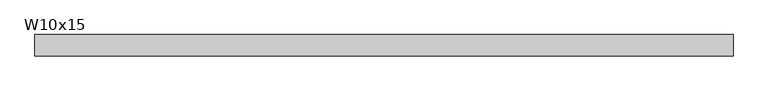
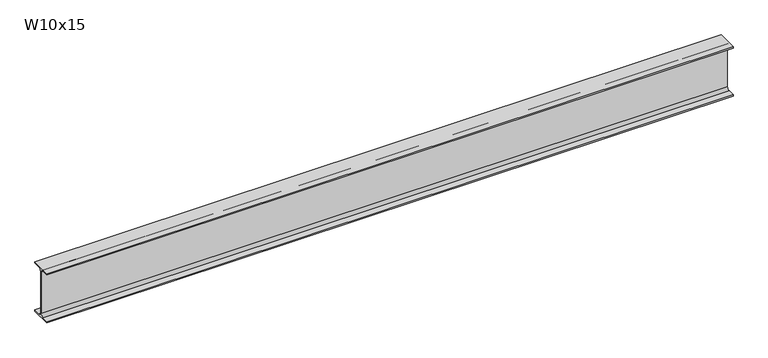
"""IFC4 building model written with IfcOpenShell, lengths in millimetres: beam geometry, RME W-Wide Flange : W10x15."""

import ifcopenshell
import ifcopenshell.guid

model = None  # the IFC model being written
_history = None  # IfcOwnerHistory: only IFC2X3 demands one
_inside = {}  # id of a spatial element -> (the spatial element, [elements in it])
_under = {}  # id of a project, library or spatial element -> (it, [spatial elements below it])
_declared = {}  # id of a project -> (the project, [libraries it declares])
_typed = {}  # id of a type object -> (the type object, [elements of that type])
_made_of = {}  # id of a material, layer set ... -> (it, [elements and type objects made of it])


def new_model(schema):
    """Start an empty IFC model of exactly this schema.

    Asked for "IFC4X3", IfcOpenShell would pick the latest addendum, in which some entities
    have other attributes; the version numbers below select the first issue.
    IFC2X3 requires an IfcOwnerHistory on every rooted entity: one is made here for all.
    """
    global model, _history
    if schema == "IFC4X3":
        model = ifcopenshell.file(schema_version=(4, 3, 0, 0))
    else:
        model = ifcopenshell.file(schema=schema)
    _inside.clear()
    _under.clear()
    _declared.clear()
    _typed.clear()
    _made_of.clear()
    _history = None
    if model.schema == "IFC2X3":
        org = make("IfcOrganization", Name="unknown")
        user = make(
            "IfcPersonAndOrganization",
            ThePerson=make("IfcPerson", FamilyName="unknown"),
            TheOrganization=org,
        )
        app = make(
            "IfcApplication",
            ApplicationDeveloper=org,
            Version="unknown",
            ApplicationFullName="unknown",
            ApplicationIdentifier="unknown",
        )
        _history = make(
            "IfcOwnerHistory",
            OwningUser=user,
            OwningApplication=app,
            ChangeAction="ADDED",
            CreationDate=0,
        )
    return model


def make(cls, **values):
    """One entity of the class cls with the attributes given. An attribute that is None is left unset."""
    return model.create_entity(
        cls, **{name: value for name, value in values.items() if value is not None}
    )


def rooted(cls, **values):
    """An entity with a GlobalId (a new one), such as an element, a storey or a relation."""
    return make(cls, GlobalId=ifcopenshell.guid.new(), OwnerHistory=_history, **values)


def si_unit(unit_type, name, prefix=None):
    """IfcSIUnit, for example si_unit("LENGTHUNIT", "METRE", prefix="MILLI")."""
    return make("IfcSIUnit", UnitType=unit_type, Prefix=prefix, Name=name)


def assignment(units):
    """IfcUnitAssignment: the units of a project."""
    return None if units is None else make("IfcUnitAssignment", Units=units)


def point(xyz):
    """IfcCartesianPoint."""
    return None if xyz is None else make("IfcCartesianPoint", Coordinates=xyz)


def direction(xyz):
    """IfcDirection."""
    return None if xyz is None else make("IfcDirection", DirectionRatios=xyz)


def frame(location, z_axis=None, x_axis=None):
    """IfcAxis2Placement3D, a coordinate frame: its origin and axes. An axis left out is left unset."""
    return make(
        "IfcAxis2Placement3D",
        Location=point(location),
        Axis=direction(z_axis),
        RefDirection=direction(x_axis),
    )


def frame_2d(location, x_axis=None):
    """IfcAxis2Placement2D, a coordinate frame in the plane: its origin and x axis."""
    return make(
        "IfcAxis2Placement2D", Location=point(location), RefDirection=direction(x_axis)
    )


def origin():
    """The frame at (0, 0, 0) with its axes left unset."""
    return frame((0.0, 0.0, 0.0))


def place(relative_to, where):
    """IfcLocalPlacement: puts the frame where relative to a parent placement (None: the world)."""
    return make(
        "IfcLocalPlacement", PlacementRelTo=relative_to, RelativePlacement=where
    )


def context(
    kind, dimensions, precision=None, world=None, true_north=None, identifier=None
):
    """IfcGeometricRepresentationContext, for example the 3D "Model" context."""
    return make(
        "IfcGeometricRepresentationContext",
        ContextIdentifier=identifier,
        ContextType=kind,
        CoordinateSpaceDimension=dimensions,
        Precision=precision,
        WorldCoordinateSystem=world,
        TrueNorth=true_north,
    )


def project(units=None, contexts=None):
    """IfcProject with its units and contexts."""
    return rooted(
        "IfcProject",
        Name="project",
        RepresentationContexts=contexts,
        UnitsInContext=assignment(units),
    )


def spatial(cls, under=None, at=None, **own):
    """A site, building, storey or space (cls), placed at a placement, below another one or the project."""
    s = rooted(cls, ObjectPlacement=at, **own)
    if under is not None:
        _under.setdefault(under.id(), (under, []))[1].append(s)
    return s


def polyline(points):
    """IfcPolyline through the points."""
    return make("IfcPolyline", Points=[point(p) for p in points])


def circle_curve(where, radius):
    """IfcCircle in the frame where."""
    return make("IfcCircle", Position=where, Radius=radius)


def trimmed(basis, trim1, trim2, sense, master):
    """IfcTrimmedCurve: the piece of a basis curve between two trims."""
    return make(
        "IfcTrimmedCurve",
        BasisCurve=basis,
        Trim1=trim1,
        Trim2=trim2,
        SenseAgreement=sense,
        MasterRepresentation=master,
    )


def segment(curve, same_sense, transition):
    """IfcCompositeCurveSegment."""
    return make(
        "IfcCompositeCurveSegment",
        Transition=transition,
        SameSense=same_sense,
        ParentCurve=curve,
    )


def composite_curve(segments, self_intersect=None):
    """IfcCompositeCurve: segments joined end to end."""
    return make("IfcCompositeCurve", Segments=segments, SelfIntersect=self_intersect)


def outline(outer, holes=None, kind="AREA"):
    """IfcArbitraryClosedProfileDef: a profile drawn as a closed curve; with holes, ...WithVoids."""
    if holes is None:
        return make("IfcArbitraryClosedProfileDef", ProfileType=kind, OuterCurve=outer)
    return make(
        "IfcArbitraryProfileDefWithVoids",
        ProfileType=kind,
        OuterCurve=outer,
        InnerCurves=holes,
    )


def extrude(swept, where, along, depth):
    """IfcExtrudedAreaSolid: the profile swept, set in the frame where, extruded along a direction by depth."""
    return make(
        "IfcExtrudedAreaSolid",
        SweptArea=swept,
        Position=where,
        ExtrudedDirection=direction(along),
        Depth=depth,
    )


def shape(context_of_items, identifier, shape_type, items):
    """IfcShapeRepresentation: the items that make up one representation, for example the "Body"."""
    return make(
        "IfcShapeRepresentation",
        ContextOfItems=context_of_items,
        RepresentationIdentifier=identifier,
        RepresentationType=shape_type,
        Items=items,
    )


def source(mapping_origin, context_of_items, identifier, shape_type, items):
    """IfcRepresentationMap: a shape defined once, which mapped items show again and again."""
    return make(
        "IfcRepresentationMap",
        MappingOrigin=mapping_origin,
        MappedRepresentation=shape(context_of_items, identifier, shape_type, items),
    )


def transform(
    local_origin,
    x_axis=None,
    y_axis=None,
    z_axis=None,
    scale=None,
    scale2=None,
    scale3=None,
    uniform=True,
):
    """IfcCartesianTransformationOperator3D, or its non-uniform kind. x_axis, y_axis, z_axis: its Axis1, 2, 3."""
    if uniform:
        return make(
            "IfcCartesianTransformationOperator3D",
            Axis1=direction(x_axis),
            Axis2=direction(y_axis),
            LocalOrigin=point(local_origin),
            Scale=scale,
            Axis3=direction(z_axis),
        )
    return make(
        "IfcCartesianTransformationOperator3DnonUniform",
        Axis1=direction(x_axis),
        Axis2=direction(y_axis),
        LocalOrigin=point(local_origin),
        Scale=scale,
        Axis3=direction(z_axis),
        Scale2=scale2,
        Scale3=scale3,
    )


def mapped(mapping_source, mapping_target):
    """IfcMappedItem: shows the shape of a source again, moved by a transform."""
    return make(
        "IfcMappedItem", MappingSource=mapping_source, MappingTarget=mapping_target
    )


def made_of(thing, what):
    """Note that an element or type object is made of a material, layer set ...; save() writes the relation."""
    if what is not None:
        _made_of.setdefault(what.id(), (what, []))[1].append(thing)
    return thing


def element(
    cls,
    number,
    at=None,
    inside=None,
    cuts=None,
    type_object=None,
    material=None,
    context=None,
    identifier="Body",
    shape_type=None,
    held_by="IfcProductDefinitionShape",
    body=None,
    shapes=None,
    **own,
):
    """One element of the class cls, such as IfcWall. Its Tag is "e" and its number.

    at: its placement. inside: the storey or other place that contains it. cuts: it is an
    opening in that element (IfcRelVoidsElement). A single representation is given by context,
    identifier, shape_type and body (its items); several are given by shapes. held_by: the class
    of the entity that holds the representations. save() writes the other relations.
    """
    e = rooted(cls, Tag="e%d" % number, ObjectPlacement=at, **own)
    if body is not None:
        shapes = [shape(context, identifier, shape_type, body)]
    if shapes is not None:
        e.Representation = make(held_by, Representations=shapes)
    if inside is not None:
        _inside.setdefault(inside.id(), (inside, []))[1].append(e)
    if cuts is not None:
        rooted(
            "IfcRelVoidsElement", RelatingBuildingElement=cuts, RelatedOpeningElement=e
        )
    if type_object is not None:
        _typed.setdefault(type_object.id(), (type_object, []))[1].append(e)
    return made_of(e, material)


def aggregate(whole, parts):
    """IfcRelAggregates: a whole, such as a stair, and the parts it consists of."""
    return rooted("IfcRelAggregates", RelatingObject=whole, RelatedObjects=parts)


def save(model, path):
    """Write the relations noted so far, then the file.

    IfcRelAggregates (storeys below a building ...), IfcRelContainedInSpatialStructure (elements
    in a storey), IfcRelDefinesByType, IfcRelAssociatesMaterial and IfcRelDeclares: one each for
    every whole, place, type object, material and project.
    """
    for whole, parts in _under.values():
        aggregate(whole, parts)
    for where, things in _inside.values():
        rooted(
            "IfcRelContainedInSpatialStructure",
            RelatedElements=things,
            RelatingStructure=where,
        )
    for kind, things in _typed.values():
        rooted("IfcRelDefinesByType", RelatedObjects=things, RelatingType=kind)
    for what, things in _made_of.values():
        rooted("IfcRelAssociatesMaterial", RelatedObjects=things, RelatingMaterial=what)
    for by, libraries in _declared.values():
        rooted("IfcRelDeclares", RelatingContext=by, RelatedDefinitions=libraries)
    model.write(path)


def w10x15_412ed89f(model_context):
    return source(origin(), model_context, "Body", "SweptSolid", [
        extrude(outline(composite_curve([segment(polyline([(50.8, -120.142), (50.8, -127.0), (-50.8, -127.0), (-50.8, -120.142), (-16.7005, -120.142)]), True, "CONTINUOUS"), segment(trimmed(circle_curve(frame_2d((-16.7005, -106.3625)), 13.7795), [point((-16.7005, -120.142))], [point((-2.921, -106.3625))], True, "CARTESIAN"), True, "CONTINUOUS"), segment(polyline([(-2.921, -106.3625), (-2.921, 106.3625)]), True, "CONTINUOUS"), segment(trimmed(circle_curve(frame_2d((-16.7005, 106.3625)), 13.7795), [point((-2.921, 106.3625))], [point((-16.7005, 120.142))], True, "CARTESIAN"), True, "CONTINUOUS"), segment(polyline([(-16.7005, 120.142), (-50.8, 120.142), (-50.8, 127.0), (50.8, 127.0), (50.8, 120.142), (16.7005, 120.142)]), True, "CONTINUOUS"), segment(trimmed(circle_curve(frame_2d((16.7005, 106.3625)), 13.7795), [point((16.7005, 120.142))], [point((2.921, 106.3625))], True, "CARTESIAN"), True, "CONTINUOUS"), segment(polyline([(2.921, 106.3625), (2.921, -106.3625)]), True, "CONTINUOUS"), segment(trimmed(circle_curve(frame_2d((16.7005, -106.3625)), 13.7795), [point((2.921, -106.3625))], [point((16.7005, -120.142))], True, "CARTESIAN"), True, "CONTINUOUS"), segment(polyline([(16.7005, -120.142), (50.8, -120.142)]), True, "CONTINUOUS")], self_intersect=False)), frame((-1681.74691, 0.0, 0.0), z_axis=(1.0, 0.0, 0.0), x_axis=(0.0, 1.0, 0.0)), (0.0, 0.0, 1.0), 3337.6914745),
    ])


if __name__ == "__main__":
    model = new_model("IFC4")
    model_context = context("Model", 3, world=origin())
    ifc_project = project(units=[si_unit("LENGTHUNIT", "METRE", prefix="MILLI")], contexts=[model_context])
    site = spatial("IfcSite", under=ifc_project)
    building = spatial("IfcBuilding", under=site)
    placement = place(None, origin())
    w10x15_shape = w10x15_412ed89f(model_context)
    element("IfcBeam", 1, ObjectType="RME W-Wide Flange : W10x15", at=placement, inside=building, context=model_context, shape_type="MappedRepresentation", body=[
        mapped(w10x15_shape, transform((0.0, 0.0, 0.0), x_axis=(1.0, 0.0, 0.0), y_axis=(0.0, 1.0, 0.0), z_axis=(0.0, 0.0, 1.0))),
    ])
    save(model, "model.ifc")

# Revit data of these elements
# Type "RME W-Wide Flange : W10x15"
#   WELD P [instance default] = ""
#   WELD LE [instance default] = ""
#   WELD D [instance default] = ""
#   TOP SECTION SIZE [instance default] = ""
#   TOP SECTION LENGTH [instance default] = ""
#   REMARKS [instance default] = ""
#   REINF TYPE [instance default] = ""
#   Nominal Size = "W24"
#   End Bearing Capacity [instance default] = ""
#   BOT SECTION SIZE [instance default] = ""
#   BOT SECTION LENGTH [instance default] = ""
#   Assembly Code = "B10"
#   W = 15
#   Start Extension Calculation [instance default] = 10' - 0"
#   Start Extension [instance default] = -0' - 0 1/2"
#   End Extension Calculation [instance default] = 10' - 0"
#   End Extension [instance default] = -0' - 0 1/2"
#   Length [instance default] = 5' - 0"
#   bf = 0' - 4"
#   d = 0' - 10"
#   k = 0' - 0 13/16"
#   k2 = 0' - 0.5425"
#   tf = 0' - 0.27"
#   tw = 0' - 0.23"
#   A = 0.030625 SF
#   Structural Material [instance default] = Metal - Steel - ASTM A992
# Element 1 (IfcBeam, "RME W-Wide Flange : W10x15")
#   Start Extension Calculation = 10' - 1.01584"
#   Start Extension = 0' - 0.51584"
#   Length = 10' - 10.38934"
#   Materials on its faces: "Metal - Steel - ASTM A992"
# Materials
#   "Metal - Steel - ASTM A992": class "Metal", colour RGB 255 128 0, transparency 0
